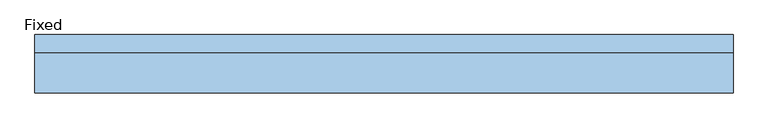
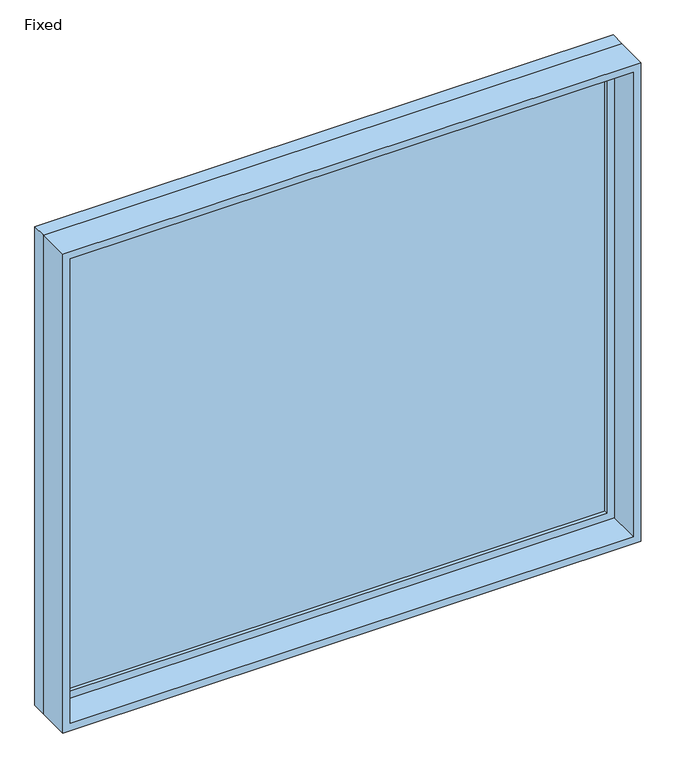
"""IFC4 building model written with IfcOpenShell, lengths in millimetres: window geometry, Fixed : dough."""

from ifc_helpers import new_model, si_unit, frame, origin, place, context, project, spatial, polyline, outline, extrude, source, transform, mapped, element, save


def fixed_de4811a9(model_context):
    return source(origin(), model_context, "Body", "SweptSolid", [
        extrude(outline(polyline([(1117.6, 53.975), (-1193.8, 53.975), (-1193.8, 66.675), (1117.6, 66.675), (1117.6, 53.975)])), frame((0.0, 0.0, 1282.7), z_axis=(0.0, 0.0, 1.0), x_axis=(1.0, 0.0, 0.0)), (0.0, 0.0, 1.0), 2006.6),
        extrude(outline(polyline([(3333.75, -1238.25), (1238.25, -1238.25), (1238.25, 1162.05), (3333.75, 1162.05), (3333.75, -1238.25)]), holes=[polyline([(3289.3, -1193.8), (3289.3, 1117.6), (1282.7, 1117.6), (1282.7, -1193.8), (3289.3, -1193.8)])]), frame((0.0, 38.1, 0.0), z_axis=(0.0, 1.0, 0.0), x_axis=(0.0, 0.0, 1.0)), (0.0, 0.0, 1.0), 44.45),
        extrude(outline(polyline([(3352.8, -1257.3), (1219.2, -1257.3), (1219.2, 1181.1), (3352.8, 1181.1), (3352.8, -1257.3)]), holes=[polyline([(3321.05, -1225.55), (3321.05, 1149.35), (1250.95, 1149.35), (1250.95, -1225.55), (3321.05, -1225.55)])]), frame((0.0, -101.6, 0.0), z_axis=(0.0, 1.0, 0.0), x_axis=(0.0, 0.0, 1.0)), (0.0, 0.0, 1.0), 139.7),
        extrude(outline(polyline([(3352.8, 1181.1), (3352.8, -1257.3), (1219.2, -1257.3), (1219.2, 1181.1), (3352.8, 1181.1)]), holes=[polyline([(3333.75, 1162.05), (1238.25, 1162.05), (1238.25, -1238.25), (3333.75, -1238.25), (3333.75, 1162.05)])]), frame((0.0, 38.1, 0.0), z_axis=(0.0, 1.0, 0.0), x_axis=(0.0, 0.0, 1.0)), (0.0, 0.0, 1.0), 63.5),
    ])


if __name__ == "__main__":
    model = new_model("IFC4")
    model_context = context("Model", 3, world=origin())
    ifc_project = project(units=[si_unit("LENGTHUNIT", "METRE", prefix="MILLI")], contexts=[model_context])
    site = spatial("IfcSite", under=ifc_project)
    building = spatial("IfcBuilding", under=site)
    placement = place(None, origin())
    fixed_shape = fixed_de4811a9(model_context)
    element("IfcWindow", 1, ObjectType="Fixed : dough", at=placement, inside=building, context=model_context, shape_type="MappedRepresentation", body=[
        mapped(fixed_shape, transform((0.0, 0.0, 0.0), x_axis=(1.0, 0.0, 0.0), y_axis=(0.0, 1.0, 0.0), z_axis=(0.0, 0.0, 1.0))),
    ])
    save(model, "model.ifc")

# Revit data of these elements
# Type "Fixed : dough"
#   Type Mark = "13"
#   Assembly Code = "B2020100"
#   Height = 7' - 0"
#   Default Sill Height = 4' - 0"
#   Width = 8' - 0"
#   Window Inset = 0' - 0 3/4"
#   Glass Pane Material = INSULATED GLAZING
#   Sash Material = Dark metal
#   Wall Closure = (empty or 0)
# Element 1 (IfcWindow, "Fixed : dough")
#   Materials on its faces: "Dark metal", "INSULATED GLAZING"
# Materials
#   "INSULATED GLAZING": class "Glass", colour RGB 236 240 239, transparency 0.42, Description = "Soda Lime Glass", Cost = 0
#   "Dark metal": class "Generic", colour RGB 44 29 29, transparency 0, Cost = 0
